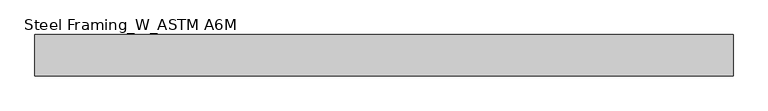
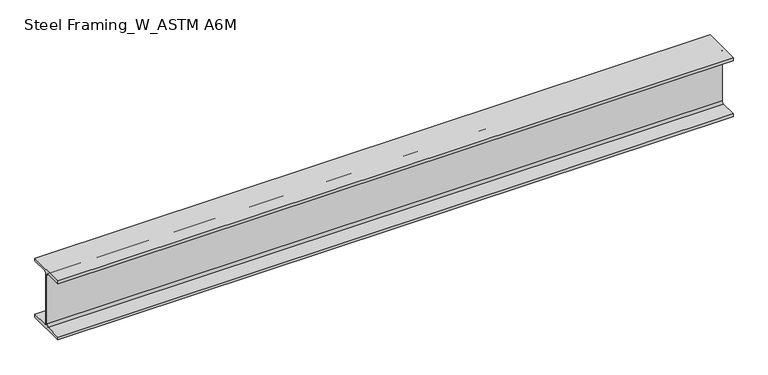
"""IFC4 building model written with IfcOpenShell, lengths in millimetres: beam geometry, Steel Framing_W_ASTM A6M : H_SB_AR_S02_W200x31.3_B6."""

from ifc_helpers import new_model, si_unit, point, frame, frame_2d, origin, place, context, project, spatial, polyline, circle_curve, trimmed, segment, composite_curve, outline, extrude, source, transform, mapped, element, save


def steel_framing_w_astm_a6m_7cdd6997(model_context):
    return source(origin(), model_context, "Body", "SweptSolid", [
        extrude(outline(composite_curve([segment(polyline([(67.0, -94.8), (67.0, -105.0), (-67.0, -105.0), (-67.0, -94.8), (-10.775, -94.8)]), True, "CONTINUOUS"), segment(trimmed(circle_curve(frame_2d((-10.775, -87.2)), 7.6), [point((-10.775, -94.8))], [point((-3.175, -87.2))], True, "CARTESIAN"), True, "CONTINUOUS"), segment(polyline([(-3.175, -87.2), (-3.175, 87.2)]), True, "CONTINUOUS"), segment(trimmed(circle_curve(frame_2d((-10.775, 87.2)), 7.6), [point((-3.175, 87.2))], [point((-10.775, 94.8))], True, "CARTESIAN"), True, "CONTINUOUS"), segment(polyline([(-10.775, 94.8), (-67.0, 94.8), (-67.0, 105.0), (67.0, 105.0), (67.0, 94.8), (10.775, 94.8)]), True, "CONTINUOUS"), segment(trimmed(circle_curve(frame_2d((10.775, 87.2)), 7.6), [point((10.775, 94.8))], [point((3.175, 87.2))], True, "CARTESIAN"), True, "CONTINUOUS"), segment(polyline([(3.175, 87.2), (3.175, -87.2)]), True, "CONTINUOUS"), segment(trimmed(circle_curve(frame_2d((10.775, -87.2)), 7.6), [point((3.175, -87.2))], [point((10.775, -94.8))], True, "CARTESIAN"), True, "CONTINUOUS"), segment(polyline([(10.775, -94.8), (67.0, -94.8)]), True, "CONTINUOUS")], self_intersect=False)), frame((-1136.3, 0.0, 0.0), z_axis=(1.0, 0.0, 0.0), x_axis=(0.0, 1.0, 0.0)), (0.0, 0.0, 1.0), 2272.1),
    ])


if __name__ == "__main__":
    model = new_model("IFC4")
    model_context = context("Model", 3, world=origin())
    ifc_project = project(units=[si_unit("LENGTHUNIT", "METRE", prefix="MILLI")], contexts=[model_context])
    site = spatial("IfcSite", under=ifc_project)
    building = spatial("IfcBuilding", under=site)
    placement = place(None, origin())
    steel_framing_w_astm_a6m_shape = steel_framing_w_astm_a6m_7cdd6997(model_context)
    element("IfcBeam", 1, ObjectType="Steel Framing_W_ASTM A6M : H_SB_AR_S02_W200x31.3_B6", at=placement, inside=building, context=model_context, shape_type="MappedRepresentation", body=[
        mapped(steel_framing_w_astm_a6m_shape, transform((0.0, 0.0, 0.0), x_axis=(1.0, 0.0, 0.0), y_axis=(0.0, 1.0, 0.0), z_axis=(0.0, 0.0, 1.0))),
    ])
    save(model, "model.ifc")

# Revit data of these elements
# Type "Steel Framing_W_ASTM A6M : H_SB_AR_S02_W200x31.3_B6"
#   Type Mark = "B6"
#   Section Name Key = "W8x21"
#   Width = 13.4 cm
#   Web Thickness = 0.635 cm
#   Web Fillet = 0.76 cm
#   Warping Constant = 40800.0 cm⁶
#   Torsional Moment of Inertia = 11.70 cm⁴
#   Section Area = 39.7 cm²
#   Plastic Modulus weak axis = 93.2 cm³
#   Plastic Modulus strong axis = 334.0 cm³
#   Perimeter = 0.93 m²/m
#   Nominal Weight = 31.30 kgf/m
#   Moment of Inertia weak axis = 407.00 cm⁴
#   Moment of Inertia strong axis = 3130.00 cm⁴
#   Height = 21.0 cm
#   Flange Thickness = 1.02 cm
#   Elastic Modulus weak axis = 60.8 cm³
#   Elastic Modulus strong axis = 298.0 cm³
#   Centroid Vertical = 10.5 cm
#   Centroid Horizontal = 6.7 cm
#   Length [instance default] = 1500 mm
#   Structural Material [instance default] = Steel, 45-345
#   Bolt Spacing = 0
#   Assembly Code = ""
# Element 1 (IfcBeam, "Steel Framing_W_ASTM A6M : H_SB_AR_S02_W200x31.3_B6")
#   Materials on its faces: "Steel, 45-345"
# Materials
#   "Steel, 45-345": class "Metal", colour RGB 189 187 185, transparency 0, Description = "Steel 345 MPa", Cost = 0
